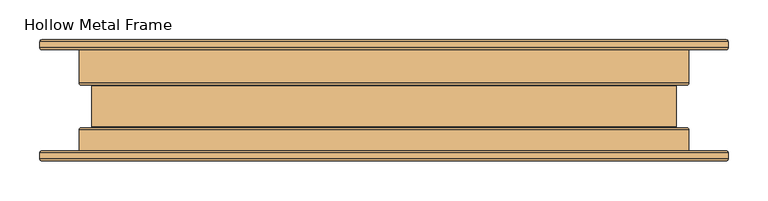
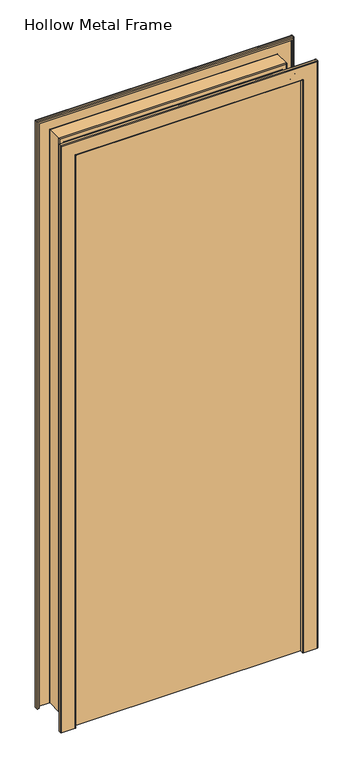
"""IFC4 building model written with IfcOpenShell, lengths in millimetres: door geometry, Hollow Metal Frame."""

import ifcopenshell
import ifcopenshell.guid

model = None  # the IFC model being written
_history = None  # IfcOwnerHistory: only IFC2X3 demands one
_inside = {}  # id of a spatial element -> (the spatial element, [elements in it])
_under = {}  # id of a project, library or spatial element -> (it, [spatial elements below it])
_declared = {}  # id of a project -> (the project, [libraries it declares])
_typed = {}  # id of a type object -> (the type object, [elements of that type])
_made_of = {}  # id of a material, layer set ... -> (it, [elements and type objects made of it])


def new_model(schema):
    """Start an empty IFC model of exactly this schema.

    Asked for "IFC4X3", IfcOpenShell would pick the latest addendum, in which some entities
    have other attributes; the version numbers below select the first issue.
    IFC2X3 requires an IfcOwnerHistory on every rooted entity: one is made here for all.
    """
    global model, _history
    if schema == "IFC4X3":
        model = ifcopenshell.file(schema_version=(4, 3, 0, 0))
    else:
        model = ifcopenshell.file(schema=schema)
    _inside.clear()
    _under.clear()
    _declared.clear()
    _typed.clear()
    _made_of.clear()
    _history = None
    if model.schema == "IFC2X3":
        org = make("IfcOrganization", Name="unknown")
        user = make(
            "IfcPersonAndOrganization",
            ThePerson=make("IfcPerson", FamilyName="unknown"),
            TheOrganization=org,
        )
        app = make(
            "IfcApplication",
            ApplicationDeveloper=org,
            Version="unknown",
            ApplicationFullName="unknown",
            ApplicationIdentifier="unknown",
        )
        _history = make(
            "IfcOwnerHistory",
            OwningUser=user,
            OwningApplication=app,
            ChangeAction="ADDED",
            CreationDate=0,
        )
    return model


def make(cls, **values):
    """One entity of the class cls with the attributes given. An attribute that is None is left unset."""
    return model.create_entity(
        cls, **{name: value for name, value in values.items() if value is not None}
    )


def rooted(cls, **values):
    """An entity with a GlobalId (a new one), such as an element, a storey or a relation."""
    return make(cls, GlobalId=ifcopenshell.guid.new(), OwnerHistory=_history, **values)


def si_unit(unit_type, name, prefix=None):
    """IfcSIUnit, for example si_unit("LENGTHUNIT", "METRE", prefix="MILLI")."""
    return make("IfcSIUnit", UnitType=unit_type, Prefix=prefix, Name=name)


def assignment(units):
    """IfcUnitAssignment: the units of a project."""
    return None if units is None else make("IfcUnitAssignment", Units=units)


def point(xyz):
    """IfcCartesianPoint."""
    return None if xyz is None else make("IfcCartesianPoint", Coordinates=xyz)


def direction(xyz):
    """IfcDirection."""
    return None if xyz is None else make("IfcDirection", DirectionRatios=xyz)


def frame(location, z_axis=None, x_axis=None):
    """IfcAxis2Placement3D, a coordinate frame: its origin and axes. An axis left out is left unset."""
    return make(
        "IfcAxis2Placement3D",
        Location=point(location),
        Axis=direction(z_axis),
        RefDirection=direction(x_axis),
    )


def origin():
    """The frame at (0, 0, 0) with its axes left unset."""
    return frame((0.0, 0.0, 0.0))


def origin_with_axes():
    """The frame at (0, 0, 0) with the z axis (0, 0, 1) and the x axis (1, 0, 0) written out."""
    return frame((0.0, 0.0, 0.0), z_axis=(0.0, 0.0, 1.0), x_axis=(1.0, 0.0, 0.0))


def place(relative_to, where):
    """IfcLocalPlacement: puts the frame where relative to a parent placement (None: the world)."""
    return make(
        "IfcLocalPlacement", PlacementRelTo=relative_to, RelativePlacement=where
    )


def context(
    kind, dimensions, precision=None, world=None, true_north=None, identifier=None
):
    """IfcGeometricRepresentationContext, for example the 3D "Model" context."""
    return make(
        "IfcGeometricRepresentationContext",
        ContextIdentifier=identifier,
        ContextType=kind,
        CoordinateSpaceDimension=dimensions,
        Precision=precision,
        WorldCoordinateSystem=world,
        TrueNorth=true_north,
    )


def project(units=None, contexts=None):
    """IfcProject with its units and contexts."""
    return rooted(
        "IfcProject",
        Name="project",
        RepresentationContexts=contexts,
        UnitsInContext=assignment(units),
    )


def spatial(cls, under=None, at=None, **own):
    """A site, building, storey or space (cls), placed at a placement, below another one or the project."""
    s = rooted(cls, ObjectPlacement=at, **own)
    if under is not None:
        _under.setdefault(under.id(), (under, []))[1].append(s)
    return s


def polyline(points):
    """IfcPolyline through the points."""
    return make("IfcPolyline", Points=[point(p) for p in points])


def circle_curve(where, radius):
    """IfcCircle in the frame where."""
    return make("IfcCircle", Position=where, Radius=radius)


def ellipse_curve(where, semi_axis1, semi_axis2):
    """IfcEllipse in the frame where."""
    return make(
        "IfcEllipse", Position=where, SemiAxis1=semi_axis1, SemiAxis2=semi_axis2
    )


def outline(outer, holes=None, kind="AREA"):
    """IfcArbitraryClosedProfileDef: a profile drawn as a closed curve; with holes, ...WithVoids."""
    if holes is None:
        return make("IfcArbitraryClosedProfileDef", ProfileType=kind, OuterCurve=outer)
    return make(
        "IfcArbitraryProfileDefWithVoids",
        ProfileType=kind,
        OuterCurve=outer,
        InnerCurves=holes,
    )


def extrude(swept, where, along, depth):
    """IfcExtrudedAreaSolid: the profile swept, set in the frame where, extruded along a direction by depth."""
    return make(
        "IfcExtrudedAreaSolid",
        SweptArea=swept,
        Position=where,
        ExtrudedDirection=direction(along),
        Depth=depth,
    )


def shape(context_of_items, identifier, shape_type, items):
    """IfcShapeRepresentation: the items that make up one representation, for example the "Body"."""
    return make(
        "IfcShapeRepresentation",
        ContextOfItems=context_of_items,
        RepresentationIdentifier=identifier,
        RepresentationType=shape_type,
        Items=items,
    )


def source(mapping_origin, context_of_items, identifier, shape_type, items):
    """IfcRepresentationMap: a shape defined once, which mapped items show again and again."""
    return make(
        "IfcRepresentationMap",
        MappingOrigin=mapping_origin,
        MappedRepresentation=shape(context_of_items, identifier, shape_type, items),
    )


def transform(
    local_origin,
    x_axis=None,
    y_axis=None,
    z_axis=None,
    scale=None,
    scale2=None,
    scale3=None,
    uniform=True,
):
    """IfcCartesianTransformationOperator3D, or its non-uniform kind. x_axis, y_axis, z_axis: its Axis1, 2, 3."""
    if uniform:
        return make(
            "IfcCartesianTransformationOperator3D",
            Axis1=direction(x_axis),
            Axis2=direction(y_axis),
            LocalOrigin=point(local_origin),
            Scale=scale,
            Axis3=direction(z_axis),
        )
    return make(
        "IfcCartesianTransformationOperator3DnonUniform",
        Axis1=direction(x_axis),
        Axis2=direction(y_axis),
        LocalOrigin=point(local_origin),
        Scale=scale,
        Axis3=direction(z_axis),
        Scale2=scale2,
        Scale3=scale3,
    )


def mapped(mapping_source, mapping_target):
    """IfcMappedItem: shows the shape of a source again, moved by a transform."""
    return make(
        "IfcMappedItem", MappingSource=mapping_source, MappingTarget=mapping_target
    )


def made_of(thing, what):
    """Note that an element or type object is made of a material, layer set ...; save() writes the relation."""
    if what is not None:
        _made_of.setdefault(what.id(), (what, []))[1].append(thing)
    return thing


def element(
    cls,
    number,
    at=None,
    inside=None,
    cuts=None,
    type_object=None,
    material=None,
    context=None,
    identifier="Body",
    shape_type=None,
    held_by="IfcProductDefinitionShape",
    body=None,
    shapes=None,
    **own,
):
    """One element of the class cls, such as IfcWall. Its Tag is "e" and its number.

    at: its placement. inside: the storey or other place that contains it. cuts: it is an
    opening in that element (IfcRelVoidsElement). A single representation is given by context,
    identifier, shape_type and body (its items); several are given by shapes. held_by: the class
    of the entity that holds the representations. save() writes the other relations.
    """
    e = rooted(cls, Tag="e%d" % number, ObjectPlacement=at, **own)
    if body is not None:
        shapes = [shape(context, identifier, shape_type, body)]
    if shapes is not None:
        e.Representation = make(held_by, Representations=shapes)
    if inside is not None:
        _inside.setdefault(inside.id(), (inside, []))[1].append(e)
    if cuts is not None:
        rooted(
            "IfcRelVoidsElement", RelatingBuildingElement=cuts, RelatedOpeningElement=e
        )
    if type_object is not None:
        _typed.setdefault(type_object.id(), (type_object, []))[1].append(e)
    return made_of(e, material)


def aggregate(whole, parts):
    """IfcRelAggregates: a whole, such as a stair, and the parts it consists of."""
    return rooted("IfcRelAggregates", RelatingObject=whole, RelatedObjects=parts)


def save(model, path):
    """Write the relations noted so far, then the file.

    IfcRelAggregates (storeys below a building ...), IfcRelContainedInSpatialStructure (elements
    in a storey), IfcRelDefinesByType, IfcRelAssociatesMaterial and IfcRelDeclares: one each for
    every whole, place, type object, material and project.
    """
    for whole, parts in _under.values():
        aggregate(whole, parts)
    for where, things in _inside.values():
        rooted(
            "IfcRelContainedInSpatialStructure",
            RelatedElements=things,
            RelatingStructure=where,
        )
    for kind, things in _typed.values():
        rooted("IfcRelDefinesByType", RelatedObjects=things, RelatingType=kind)
    for what, things in _made_of.values():
        rooted("IfcRelAssociatesMaterial", RelatedObjects=things, RelatingMaterial=what)
    for by, libraries in _declared.values():
        rooted("IfcRelDeclares", RelatingContext=by, RelatedDefinitions=libraries)
    model.write(path)


def plane_surface(at):
    """IfcPlane: the flat surface through the origin of the frame at, square to its z axis."""
    return make("IfcPlane", Position=at)


def cylinder_surface(at, radius):
    """IfcCylindricalSurface: all points at the distance radius from the z axis of the frame at."""
    return make("IfcCylindricalSurface", Position=at, Radius=radius)


def revolved_surface(curve, axis_point, axis_direction):
    """IfcSurfaceOfRevolution: the curve turned about the line through axis_point along axis_direction."""
    return make(
        "IfcSurfaceOfRevolution",
        SweptCurve=make("IfcArbitraryOpenProfileDef", ProfileType="CURVE", Curve=curve),
        AxisPosition=make("IfcAxis1Placement", Location=point(axis_point), Axis=direction(axis_direction)),
    )


def advanced_brep(points, edges, surfaces, faces):
    """IfcAdvancedBrep: a solid bounded by faces that lie on surfaces and meet in shared edges.

    An edge is (start, end): straight between two places in points (the first is 0);
    or (start, end, curve); or (start, end, curve, False) where it runs against its curve.
    A face is (place in surfaces, loops), or (place, loops, False) where it looks against
    its surface's normal. A loop lists edges by number (the first is 1), with a minus sign
    where the edge is run from its end to its start. The first loop is the outer one.
    """
    corners = [point(p) for p in points]
    vertices = [make("IfcVertexPoint", VertexGeometry=c) for c in corners]
    made = []
    for start, end, *more in edges:
        made.append(
            make(
                "IfcEdgeCurve",
                EdgeStart=vertices[start],
                EdgeEnd=vertices[end],
                EdgeGeometry=more[0] if more else make("IfcPolyline", Points=[corners[start], corners[end]]),
                SameSense=more[1] if len(more) > 1 else True,
            )
        )
    hull = []
    for where, loops, *sense in faces:
        bounds = []
        for j, loop in enumerate(loops):
            ring = [make("IfcOrientedEdge", EdgeElement=made[abs(k) - 1], Orientation=k > 0) for k in loop]
            bounds.append(
                make(
                    "IfcFaceOuterBound" if j == 0 else "IfcFaceBound",
                    Bound=make("IfcEdgeLoop", EdgeList=ring),
                    Orientation=True,
                )
            )
        hull.append(make("IfcAdvancedFace", Bounds=bounds, FaceSurface=surfaces[where], SameSense=sense[0] if sense else True))
    return make("IfcAdvancedBrep", Outer=make("IfcClosedShell", CfsFaces=hull))


def hollow_metal_frame_ce1c65a4(model_context):
    return source(origin(), model_context, "Body", "SolidModel", [
        advanced_brep(
        [(-429.22825, 63.5635, 0.0), (-431.8, 66.13525, 0.0), (-431.8, 73.66, 0.0), (-429.22825, 76.23175, 0.0), (-383.57175, 76.23175, 0.0), (-381.0, 73.66, 0.0), (-381.0, 21.68525, 0.0), (-379.984, 20.66925, 0.0), (-367.69675, 20.66925, 0.0), (-365.125, 18.0975, 0.0), (-365.125, -33.6931, 0.0), (-367.69675, -36.26485, 0.0), (-379.984, -36.26485, 0.0), (-381.0, -37.28085, 0.0), (-381.0, -73.5965, 0.0), (-383.57175, -76.16825, 0.0), (-429.22825, -76.16825, 0.0), (-431.8, -73.5965, 0.0), (-431.8, -66.07175, 0.0), (-429.22825, -63.5, 0.0), (-423.8625, -63.5, 0.0), (-423.8625, -65.05575, 0.0), (-429.22825, -65.05575, 0.0), (-430.24425, -66.07175, 0.0), (-430.24425, -73.5965, 0.0), (-429.22825, -74.6125, 0.0), (-383.57175, -74.6125, 0.0), (-382.55575, -73.5965, 0.0), (-382.55575, -37.28085, 0.0), (-379.984, -34.7091, 0.0), (-367.69675, -34.7091, 0.0), (-366.68075, -33.6931, 0.0), (-366.68075, 18.0975, 0.0), (-367.69675, 19.1135, 0.0), (-379.984, 19.1135, 0.0), (-382.55575, 21.68525, 0.0), (-382.55575, 73.66, 0.0), (-383.57175, 74.676, 0.0), (-429.22825, 74.676, 0.0), (-430.24425, 73.66, 0.0), (-430.24425, 66.13525, 0.0), (-429.22825, 65.11925, 0.0), (-423.8625, 65.11925, 0.0), (-423.8625, 63.5635, 0.0), (-429.22825, 63.5635, 2080.2282501), (-431.8, 66.13525, 2082.8000001), (-431.8, 73.66, 2082.8000001), (-429.22825, 76.23175, 2080.2282501), (429.22825, 76.23175, 2080.2282501), (429.22825, 76.23175, 0.0), (383.57175, 76.23175, 0.0), (383.57175, 76.23175, 2034.5717501), (-383.57175, 76.23175, 2034.5717501), (-381.0, 73.66, 2032.0000001), (-381.0, 21.68525, 2032.0000001), (-379.984, 20.66925, 2030.9840001), (379.984, 20.66925, 2030.9840001), (379.984, 20.66925, 0.0), (367.69675, 20.66925, 0.0), (367.69675, 20.66925, 2018.6967501), (-367.69675, 20.66925, 2018.6967501), (-365.125, 18.0975, 2016.1250001), (-365.125, -33.6931, 2016.1250001), (-367.69675, -36.26485, 2018.6967501), (367.69675, -36.26485, 2018.6967501), (367.69675, -36.26485, 0.0), (379.984, -36.26485, 0.0), (379.984, -36.26485, 2030.9840001), (-379.984, -36.26485, 2030.9840001), (-381.0, -37.28085, 2032.0000001), (-381.0, -73.5965, 2032.0000001), (-383.57175, -76.16825, 2034.5717501), (383.57175, -76.16825, 2034.5717501), (383.57175, -76.16825, 0.0), (429.22825, -76.16825, 0.0), (429.22825, -76.16825, 2080.2282501), (-429.22825, -76.16825, 2080.2282501), (-431.8, -73.5965, 2082.8000001), (-431.8, -66.07175, 2082.8000001), (-429.22825, -63.5, 2080.2282501), (429.22825, -63.5, 2080.2282501), (429.22825, -63.5, 0.0), (423.8625, -63.5, 0.0), (423.8625, -63.5, 2074.8625001), (-423.8625, -63.5, 2074.8625001), (-423.8625, -65.05575, 2074.8625001), (423.8625, -65.05575, 2074.8625001), (423.8625, -65.05575, 0.0), (429.22825, -65.05575, 0.0), (429.22825, -65.05575, 2080.2282501), (-429.22825, -65.05575, 2080.2282501), (-430.24425, -66.07175, 2081.2442501), (-430.24425, -73.5965, 2081.2442501), (-429.22825, -74.6125, 2080.2282501), (429.22825, -74.6125, 2080.2282501), (429.22825, -74.6125, 0.0), (383.57175, -74.6125, 0.0), (383.57175, -74.6125, 2034.5717501), (-383.57175, -74.6125, 2034.5717501), (-382.55575, -73.5965, 2033.5557501), (-382.55575, -37.28085, 2033.5557501), (-379.984, -34.7091, 2030.9840001), (379.984, -34.7091, 2030.9840001), (379.984, -34.7091, 0.0), (367.69675, -34.7091, 0.0), (367.69675, -34.7091, 2018.6967501), (-367.69675, -34.7091, 2018.6967501), (-366.68075, -33.6931, 2017.6807501), (-366.68075, 18.0975, 2017.6807501), (-367.69675, 19.1135, 2018.6967501), (367.69675, 19.1135, 2018.6967501), (367.69675, 19.1135, 0.0), (379.984, 19.1135, 0.0), (379.984, 19.1135, 2030.9840001), (-379.984, 19.1135, 2030.9840001), (-382.55575, 21.68525, 2033.5557501), (-382.55575, 73.66, 2033.5557501), (-383.57175, 74.676, 2034.5717501), (383.57175, 74.676, 2034.5717501), (383.57175, 74.676, 0.0), (429.22825, 74.676, 0.0), (429.22825, 74.676, 2080.2282501), (-429.22825, 74.676, 2080.2282501), (-430.24425, 73.66, 2081.2442501), (-430.24425, 66.13525, 2081.2442501), (-429.22825, 65.11925, 2080.2282501), (429.22825, 65.11925, 2080.2282501), (429.22825, 65.11925, 0.0), (423.8625, 65.11925, 0.0), (423.8625, 65.11925, 2074.8625001), (-423.8625, 65.11925, 2074.8625001), (-423.8625, 63.5635, 2074.8625001), (423.8625, 63.5635, 2074.8625001), (423.8625, 63.5635, 0.0), (429.22825, 63.5635, 0.0), (429.22825, 63.5635, 2080.2282501), (431.8, 66.13525, 2082.8000001), (431.8, 73.66, 2082.8000001), (381.0, 73.66, 2032.0000001), (381.0, 21.68525, 2032.0000001), (365.125, 18.0975, 2016.1250001), (365.125, -33.6931, 2016.1250001), (381.0, -37.28085, 2032.0000001), (381.0, -73.5965, 2032.0000001), (431.8, -73.5965, 2082.8000001), (431.8, -66.07175, 2082.8000001), (430.24425, -66.07175, 2081.2442501), (430.24425, -73.5965, 2081.2442501), (382.55575, -73.5965, 2033.5557501), (382.55575, -37.28085, 2033.5557501), (366.68075, -33.6931, 2017.6807501), (366.68075, 18.0975, 2017.6807501), (382.55575, 21.68525, 2033.5557501), (382.55575, 73.66, 2033.5557501), (430.24425, 73.66, 2081.2442501), (430.24425, 66.13525, 2081.2442501), (430.24425, 66.13525, 0.0), (430.24425, 73.66, 0.0), (382.55575, 73.66, 0.0), (382.55575, 21.68525, 0.0), (366.68075, 18.0975, 0.0), (366.68075, -33.6931, 0.0), (382.55575, -37.28085, 0.0), (382.55575, -73.5965, 0.0), (430.24425, -73.5965, 0.0), (430.24425, -66.07175, 0.0), (431.8, -66.07175, 0.0), (431.8, -73.5965, 0.0), (381.0, -73.5965, 0.0), (381.0, -37.28085, 0.0), (365.125, -33.6931, 0.0), (365.125, 18.0975, 0.0), (381.0, 21.68525, 0.0), (381.0, 73.66, 0.0), (431.8, 73.66, 0.0), (431.8, 66.13525, 0.0)],
        [
            (0, 1, circle_curve(frame((-429.22825, 66.13525, 0.0), z_axis=(0.0, 0.0, -1.0), x_axis=(0.0, -1.0, 0.0)), 2.57175)),
            (1, 2),
            (2, 3, circle_curve(frame((-429.22825, 73.66, 0.0), z_axis=(0.0, 0.0, -1.0), x_axis=(0.0, -1.0, 0.0)), 2.57175)),
            (3, 4),
            (4, 5, circle_curve(frame((-383.57175, 73.66, 0.0), z_axis=(0.0, 0.0, -1.0), x_axis=(0.0, -1.0, 0.0)), 2.57175)),
            (5, 6),
            (6, 7, circle_curve(frame((-379.984, 21.68525, 0.0), z_axis=(0.0, 0.0, 1.0), x_axis=(0.0, -1.0, 0.0)), 1.016)),
            (7, 8),
            (8, 9, circle_curve(frame((-367.69675, 18.0975, 0.0), z_axis=(0.0, 0.0, -1.0), x_axis=(0.0, -1.0, 0.0)), 2.57175)),
            (9, 10),
            (10, 11, circle_curve(frame((-367.69675, -33.6931, 0.0), z_axis=(0.0, 0.0, -1.0), x_axis=(0.0, -1.0, 0.0)), 2.57175)),
            (11, 12),
            (12, 13, circle_curve(frame((-379.984, -37.28085, 0.0), z_axis=(0.0, 0.0, 1.0), x_axis=(0.0, -1.0, 0.0)), 1.016)),
            (13, 14),
            (14, 15, circle_curve(frame((-383.57175, -73.5965, 0.0), z_axis=(0.0, 0.0, -1.0), x_axis=(0.0, -1.0, 0.0)), 2.57175)),
            (15, 16),
            (16, 17, circle_curve(frame((-429.22825, -73.5965, 0.0), z_axis=(0.0, 0.0, -1.0), x_axis=(0.0, -1.0, 0.0)), 2.57175)),
            (17, 18),
            (18, 19, circle_curve(frame((-429.22825, -66.07175, 0.0), z_axis=(0.0, 0.0, -1.0), x_axis=(0.0, -1.0, 0.0)), 2.57175)),
            (19, 20),
            (20, 21),
            (21, 22),
            (22, 23, circle_curve(frame((-429.22825, -66.07175, 0.0), z_axis=(0.0, 0.0, 1.0), x_axis=(0.0, -1.0, 0.0)), 1.016)),
            (23, 24),
            (24, 25, circle_curve(frame((-429.22825, -73.5965, 0.0), z_axis=(0.0, 0.0, 1.0), x_axis=(0.0, -1.0, 0.0)), 1.016)),
            (25, 26),
            (26, 27, circle_curve(frame((-383.57175, -73.5965, 0.0), z_axis=(0.0, 0.0, 1.0), x_axis=(0.0, -1.0, 0.0)), 1.016)),
            (27, 28),
            (28, 29, circle_curve(frame((-379.984, -37.28085, 0.0), z_axis=(0.0, 0.0, -1.0), x_axis=(0.0, -1.0, 0.0)), 2.57175)),
            (29, 30),
            (30, 31, circle_curve(frame((-367.69675, -33.6931, 0.0), z_axis=(0.0, 0.0, 1.0), x_axis=(0.0, -1.0, 0.0)), 1.016)),
            (31, 32),
            (32, 33, circle_curve(frame((-367.69675, 18.0975, 0.0), z_axis=(0.0, 0.0, 1.0), x_axis=(0.0, -1.0, 0.0)), 1.016)),
            (33, 34),
            (34, 35, circle_curve(frame((-379.984, 21.68525, 0.0), z_axis=(0.0, 0.0, -1.0), x_axis=(0.0, -1.0, 0.0)), 2.57175)),
            (35, 36),
            (36, 37, circle_curve(frame((-383.57175, 73.66, 0.0), z_axis=(0.0, 0.0, 1.0), x_axis=(0.0, -1.0, 0.0)), 1.016)),
            (37, 38),
            (38, 39, circle_curve(frame((-429.22825, 73.66, 0.0), z_axis=(0.0, 0.0, 1.0), x_axis=(0.0, -1.0, 0.0)), 1.016)),
            (39, 40),
            (40, 41, circle_curve(frame((-429.22825, 66.13525, 0.0), z_axis=(0.0, 0.0, 1.0), x_axis=(0.0, -1.0, 0.0)), 1.016)),
            (41, 42),
            (42, 43),
            (43, 0),
            (0, 44),
            (44, 45, ellipse_curve(frame((-429.22825, 66.13525, 2080.2282501), z_axis=(-0.7071067811865475, 0.0, -0.7071067811865475), x_axis=(0.7071067811865474, 0.0, -0.7071067811865476)), 3.6370037, 2.57175)),
            (45, 1),
            (45, 46),
            (46, 2),
            (46, 47, ellipse_curve(frame((-429.22825, 73.66, 2080.2282501), z_axis=(-0.7071067811865475, 0.0, -0.7071067811865475), x_axis=(0.7071067811865474, 0.0, -0.7071067811865476)), 3.6370037, 2.57175)),
            (47, 3),
            (47, 48),
            (48, 49),
            (49, 50),
            (50, 51),
            (51, 52),
            (52, 4),
            (52, 53, ellipse_curve(frame((-383.57175, 73.66, 2034.5717501), z_axis=(-0.7071067811865475, 0.0, -0.7071067811865475), x_axis=(0.7071067811865474, 0.0, -0.7071067811865476)), 3.6370037, 2.57175)),
            (53, 5),
            (53, 54),
            (54, 6),
            (54, 55, ellipse_curve(frame((-379.984, 21.68525, 2030.9840001), z_axis=(0.7071067811865475, 0.0, 0.7071067811865475), x_axis=(-0.7071067811865474, 0.0, 0.7071067811865476)), 1.436841, 1.016)),
            (55, 7),
            (55, 56),
            (56, 57),
            (57, 58),
            (58, 59),
            (59, 60),
            (60, 8),
            (60, 61, ellipse_curve(frame((-367.69675, 18.0975, 2018.6967501), z_axis=(-0.7071067811865475, 0.0, -0.7071067811865475), x_axis=(0.7071067811865474, 0.0, -0.7071067811865476)), 3.6370037, 2.57175)),
            (61, 9),
            (61, 62),
            (62, 10),
            (62, 63, ellipse_curve(frame((-367.69675, -33.6931, 2018.6967501), z_axis=(-0.7071067811865475, 0.0, -0.7071067811865475), x_axis=(0.7071067811865474, 0.0, -0.7071067811865476)), 3.6370037, 2.57175)),
            (63, 11),
            (63, 64),
            (64, 65),
            (65, 66),
            (66, 67),
            (67, 68),
            (68, 12),
            (68, 69, ellipse_curve(frame((-379.984, -37.28085, 2030.9840001), z_axis=(0.7071067811865475, 0.0, 0.7071067811865475), x_axis=(-0.7071067811865474, 0.0, 0.7071067811865476)), 1.436841, 1.016)),
            (69, 13),
            (69, 70),
            (70, 14),
            (70, 71, ellipse_curve(frame((-383.57175, -73.5965, 2034.5717501), z_axis=(-0.7071067811865475, 0.0, -0.7071067811865475), x_axis=(0.7071067811865474, 0.0, -0.7071067811865476)), 3.6370037, 2.57175)),
            (71, 15),
            (71, 72),
            (72, 73),
            (73, 74),
            (74, 75),
            (75, 76),
            (76, 16),
            (76, 77, ellipse_curve(frame((-429.22825, -73.5965, 2080.2282501), z_axis=(-0.7071067811865475, 0.0, -0.7071067811865475), x_axis=(0.7071067811865474, 0.0, -0.7071067811865476)), 3.6370037, 2.57175)),
            (77, 17),
            (77, 78),
            (78, 18),
            (78, 79, ellipse_curve(frame((-429.22825, -66.07175, 2080.2282501), z_axis=(-0.7071067811865475, 0.0, -0.7071067811865475), x_axis=(0.7071067811865474, 0.0, -0.7071067811865476)), 3.6370037, 2.57175)),
            (79, 19),
            (79, 80),
            (80, 81),
            (81, 82),
            (82, 83),
            (83, 84),
            (84, 20),
            (84, 85),
            (85, 21),
            (85, 86),
            (86, 87),
            (87, 88),
            (88, 89),
            (89, 90),
            (90, 22),
            (90, 91, ellipse_curve(frame((-429.22825, -66.07175, 2080.2282501), z_axis=(0.7071067811865475, 0.0, 0.7071067811865475), x_axis=(-0.7071067811865474, 0.0, 0.7071067811865476)), 1.436841, 1.016)),
            (91, 23),
            (91, 92),
            (92, 24),
            (92, 93, ellipse_curve(frame((-429.22825, -73.5965, 2080.2282501), z_axis=(0.7071067811865475, 0.0, 0.7071067811865475), x_axis=(-0.7071067811865474, 0.0, 0.7071067811865476)), 1.436841, 1.016)),
            (93, 25),
            (93, 94),
            (94, 95),
            (95, 96),
            (96, 97),
            (97, 98),
            (98, 26),
            (98, 99, ellipse_curve(frame((-383.57175, -73.5965, 2034.5717501), z_axis=(0.7071067811865475, 0.0, 0.7071067811865475), x_axis=(-0.7071067811865474, 0.0, 0.7071067811865476)), 1.436841, 1.016)),
            (99, 27),
            (99, 100),
            (100, 28),
            (100, 101, ellipse_curve(frame((-379.984, -37.28085, 2030.9840001), z_axis=(-0.7071067811865475, 0.0, -0.7071067811865475), x_axis=(0.7071067811865474, 0.0, -0.7071067811865476)), 3.6370037, 2.57175)),
            (101, 29),
            (101, 102),
            (102, 103),
            (103, 104),
            (104, 105),
            (105, 106),
            (106, 30),
            (106, 107, ellipse_curve(frame((-367.69675, -33.6931, 2018.6967501), z_axis=(0.7071067811865475, 0.0, 0.7071067811865475), x_axis=(-0.7071067811865474, 0.0, 0.7071067811865476)), 1.436841, 1.016)),
            (107, 31),
            (107, 108),
            (108, 32),
            (108, 109, ellipse_curve(frame((-367.69675, 18.0975, 2018.6967501), z_axis=(0.7071067811865475, 0.0, 0.7071067811865475), x_axis=(-0.7071067811865474, 0.0, 0.7071067811865476)), 1.436841, 1.016)),
            (109, 33),
            (109, 110),
            (110, 111),
            (111, 112),
            (112, 113),
            (113, 114),
            (114, 34),
            (114, 115, ellipse_curve(frame((-379.984, 21.68525, 2030.9840001), z_axis=(-0.7071067811865475, 0.0, -0.7071067811865475), x_axis=(0.7071067811865474, 0.0, -0.7071067811865476)), 3.6370037, 2.57175)),
            (115, 35),
            (115, 116),
            (116, 36),
            (116, 117, ellipse_curve(frame((-383.57175, 73.66, 2034.5717501), z_axis=(0.7071067811865475, 0.0, 0.7071067811865475), x_axis=(-0.7071067811865474, 0.0, 0.7071067811865476)), 1.436841, 1.016)),
            (117, 37),
            (117, 118),
            (118, 119),
            (119, 120),
            (120, 121),
            (121, 122),
            (122, 38),
            (122, 123, ellipse_curve(frame((-429.22825, 73.66, 2080.2282501), z_axis=(0.7071067811865475, 0.0, 0.7071067811865475), x_axis=(-0.7071067811865474, 0.0, 0.7071067811865476)), 1.436841, 1.016)),
            (123, 39),
            (123, 124),
            (124, 40),
            (124, 125, ellipse_curve(frame((-429.22825, 66.13525, 2080.2282501), z_axis=(0.7071067811865475, 0.0, 0.7071067811865475), x_axis=(-0.7071067811865474, 0.0, 0.7071067811865476)), 1.436841, 1.016)),
            (125, 41),
            (125, 126),
            (126, 127),
            (127, 128),
            (128, 129),
            (129, 130),
            (130, 42),
            (130, 131),
            (131, 43),
            (131, 132),
            (132, 133),
            (133, 134),
            (134, 135),
            (135, 44),
            (135, 136, ellipse_curve(frame((429.22825, 66.13525, 2080.2282501), z_axis=(-0.7071067811865475, 0.0, 0.7071067811865475), x_axis=(-0.7071067811865476, 0.0, -0.7071067811865474)), 3.6370037, 2.57175)),
            (136, 45),
            (136, 137),
            (137, 46),
            (137, 48, ellipse_curve(frame((429.22825, 73.66, 2080.2282501), z_axis=(-0.7071067811865475, 0.0, 0.7071067811865475), x_axis=(-0.7071067811865476, 0.0, -0.7071067811865474)), 3.6370037, 2.57175)),
            (51, 138, ellipse_curve(frame((383.57175, 73.66, 2034.5717501), z_axis=(-0.7071067811865475, 0.0, 0.7071067811865475), x_axis=(-0.7071067811865476, 0.0, -0.7071067811865474)), 3.6370037, 2.57175)),
            (138, 53),
            (138, 139),
            (139, 54),
            (139, 56, ellipse_curve(frame((379.984, 21.68525, 2030.9840001), z_axis=(0.7071067811865475, 0.0, -0.7071067811865475), x_axis=(0.7071067811865476, 0.0, 0.7071067811865474)), 1.436841, 1.016)),
            (59, 140, ellipse_curve(frame((367.69675, 18.0975, 2018.6967501), z_axis=(-0.7071067811865475, 0.0, 0.7071067811865475), x_axis=(-0.7071067811865476, 0.0, -0.7071067811865474)), 3.6370037, 2.57175)),
            (140, 61),
            (140, 141),
            (141, 62),
            (141, 64, ellipse_curve(frame((367.69675, -33.6931, 2018.6967501), z_axis=(-0.7071067811865475, 0.0, 0.7071067811865475), x_axis=(-0.7071067811865476, 0.0, -0.7071067811865474)), 3.6370037, 2.57175)),
            (67, 142, ellipse_curve(frame((379.984, -37.28085, 2030.9840001), z_axis=(0.7071067811865475, 0.0, -0.7071067811865475), x_axis=(0.7071067811865476, 0.0, 0.7071067811865474)), 1.436841, 1.016)),
            (142, 69),
            (142, 143),
            (143, 70),
            (143, 72, ellipse_curve(frame((383.57175, -73.5965, 2034.5717501), z_axis=(-0.7071067811865475, 0.0, 0.7071067811865475), x_axis=(-0.7071067811865476, 0.0, -0.7071067811865474)), 3.6370037, 2.57175)),
            (75, 144, ellipse_curve(frame((429.22825, -73.5965, 2080.2282501), z_axis=(-0.7071067811865475, 0.0, 0.7071067811865475), x_axis=(-0.7071067811865476, 0.0, -0.7071067811865474)), 3.6370037, 2.57175)),
            (144, 77),
            (144, 145),
            (145, 78),
            (145, 80, ellipse_curve(frame((429.22825, -66.07175, 2080.2282501), z_axis=(-0.7071067811865475, 0.0, 0.7071067811865475), x_axis=(-0.7071067811865476, 0.0, -0.7071067811865474)), 3.6370037, 2.57175)),
            (83, 86),
            (89, 146, ellipse_curve(frame((429.22825, -66.07175, 2080.2282501), z_axis=(0.7071067811865475, 0.0, -0.7071067811865475), x_axis=(0.7071067811865476, 0.0, 0.7071067811865474)), 1.436841, 1.016)),
            (146, 91),
            (146, 147),
            (147, 92),
            (147, 94, ellipse_curve(frame((429.22825, -73.5965, 2080.2282501), z_axis=(0.7071067811865475, 0.0, -0.7071067811865475), x_axis=(0.7071067811865476, 0.0, 0.7071067811865474)), 1.436841, 1.016)),
            (97, 148, ellipse_curve(frame((383.57175, -73.5965, 2034.5717501), z_axis=(0.7071067811865475, 0.0, -0.7071067811865475), x_axis=(0.7071067811865476, 0.0, 0.7071067811865474)), 1.436841, 1.016)),
            (148, 99),
            (148, 149),
            (149, 100),
            (149, 102, ellipse_curve(frame((379.984, -37.28085, 2030.9840001), z_axis=(-0.7071067811865475, 0.0, 0.7071067811865475), x_axis=(-0.7071067811865476, 0.0, -0.7071067811865474)), 3.6370037, 2.57175)),
            (105, 150, ellipse_curve(frame((367.69675, -33.6931, 2018.6967501), z_axis=(0.7071067811865475, 0.0, -0.7071067811865475), x_axis=(0.7071067811865476, 0.0, 0.7071067811865474)), 1.436841, 1.016)),
            (150, 107),
            (150, 151),
            (151, 108),
            (151, 110, ellipse_curve(frame((367.69675, 18.0975, 2018.6967501), z_axis=(0.7071067811865475, 0.0, -0.7071067811865475), x_axis=(0.7071067811865476, 0.0, 0.7071067811865474)), 1.436841, 1.016)),
            (113, 152, ellipse_curve(frame((379.984, 21.68525, 2030.9840001), z_axis=(-0.7071067811865475, 0.0, 0.7071067811865475), x_axis=(-0.7071067811865476, 0.0, -0.7071067811865474)), 3.6370037, 2.57175)),
            (152, 115),
            (152, 153),
            (153, 116),
            (153, 118, ellipse_curve(frame((383.57175, 73.66, 2034.5717501), z_axis=(0.7071067811865475, 0.0, -0.7071067811865475), x_axis=(0.7071067811865476, 0.0, 0.7071067811865474)), 1.436841, 1.016)),
            (121, 154, ellipse_curve(frame((429.22825, 73.66, 2080.2282501), z_axis=(0.7071067811865475, 0.0, -0.7071067811865475), x_axis=(0.7071067811865476, 0.0, 0.7071067811865474)), 1.436841, 1.016)),
            (154, 123),
            (154, 155),
            (155, 124),
            (155, 126, ellipse_curve(frame((429.22825, 66.13525, 2080.2282501), z_axis=(0.7071067811865475, 0.0, -0.7071067811865475), x_axis=(0.7071067811865476, 0.0, 0.7071067811865474)), 1.436841, 1.016)),
            (129, 132),
            (133, 128),
            (127, 156, circle_curve(frame((429.22825, 66.13525, 0.0), z_axis=(0.0, 0.0, 1.0), x_axis=(0.0, -1.0, 0.0)), 1.016)),
            (156, 157),
            (157, 120, circle_curve(frame((429.22825, 73.66, 0.0), z_axis=(0.0, 0.0, 1.0), x_axis=(0.0, -1.0, 0.0)), 1.016)),
            (119, 158, circle_curve(frame((383.57175, 73.66, 0.0), z_axis=(0.0, 0.0, 1.0), x_axis=(0.0, -1.0, 0.0)), 1.016)),
            (158, 159),
            (159, 112, circle_curve(frame((379.984, 21.68525, 0.0), z_axis=(0.0, 0.0, -1.0), x_axis=(0.0, -1.0, 0.0)), 2.57175)),
            (111, 160, circle_curve(frame((367.69675, 18.0975, 0.0), z_axis=(0.0, 0.0, 1.0), x_axis=(0.0, -1.0, 0.0)), 1.016)),
            (160, 161),
            (161, 104, circle_curve(frame((367.69675, -33.6931, 0.0), z_axis=(0.0, 0.0, 1.0), x_axis=(0.0, -1.0, 0.0)), 1.016)),
            (103, 162, circle_curve(frame((379.984, -37.28085, 0.0), z_axis=(0.0, 0.0, -1.0), x_axis=(0.0, -1.0, 0.0)), 2.57175)),
            (162, 163),
            (163, 96, circle_curve(frame((383.57175, -73.5965, 0.0), z_axis=(0.0, 0.0, 1.0), x_axis=(0.0, -1.0, 0.0)), 1.016)),
            (95, 164, circle_curve(frame((429.22825, -73.5965, 0.0), z_axis=(0.0, 0.0, 1.0), x_axis=(0.0, -1.0, 0.0)), 1.016)),
            (164, 165),
            (165, 88, circle_curve(frame((429.22825, -66.07175, 0.0), z_axis=(0.0, 0.0, 1.0), x_axis=(0.0, -1.0, 0.0)), 1.016)),
            (87, 82),
            (81, 166, circle_curve(frame((429.22825, -66.07175, 0.0), z_axis=(0.0, 0.0, -1.0), x_axis=(0.0, -1.0, 0.0)), 2.57175)),
            (166, 167),
            (167, 74, circle_curve(frame((429.22825, -73.5965, 0.0), z_axis=(0.0, 0.0, -1.0), x_axis=(0.0, -1.0, 0.0)), 2.57175)),
            (73, 168, circle_curve(frame((383.57175, -73.5965, 0.0), z_axis=(0.0, 0.0, -1.0), x_axis=(0.0, -1.0, 0.0)), 2.57175)),
            (168, 169),
            (169, 66, circle_curve(frame((379.984, -37.28085, 0.0), z_axis=(0.0, 0.0, 1.0), x_axis=(0.0, -1.0, 0.0)), 1.016)),
            (65, 170, circle_curve(frame((367.69675, -33.6931, 0.0), z_axis=(0.0, 0.0, -1.0), x_axis=(0.0, -1.0, 0.0)), 2.57175)),
            (170, 171),
            (171, 58, circle_curve(frame((367.69675, 18.0975, 0.0), z_axis=(0.0, 0.0, -1.0), x_axis=(0.0, -1.0, 0.0)), 2.57175)),
            (57, 172, circle_curve(frame((379.984, 21.68525, 0.0), z_axis=(0.0, 0.0, 1.0), x_axis=(0.0, -1.0, 0.0)), 1.016)),
            (172, 173),
            (173, 50, circle_curve(frame((383.57175, 73.66, 0.0), z_axis=(0.0, 0.0, -1.0), x_axis=(0.0, -1.0, 0.0)), 2.57175)),
            (49, 174, circle_curve(frame((429.22825, 73.66, 0.0), z_axis=(0.0, 0.0, -1.0), x_axis=(0.0, -1.0, 0.0)), 2.57175)),
            (174, 175),
            (175, 134, circle_curve(frame((429.22825, 66.13525, 0.0), z_axis=(0.0, 0.0, -1.0), x_axis=(0.0, -1.0, 0.0)), 2.57175)),
            (175, 136),
            (174, 137),
            (173, 138),
            (172, 139),
            (171, 140),
            (170, 141),
            (169, 142),
            (168, 143),
            (167, 144),
            (166, 145),
            (165, 146),
            (164, 147),
            (163, 148),
            (162, 149),
            (161, 150),
            (160, 151),
            (159, 152),
            (158, 153),
            (157, 154),
            (156, 155),
        ],
        [
            plane_surface(frame((-392.1125, -63.5, 0.0), z_axis=(0.0, 0.0, -1.0), x_axis=(1.0, 0.0, 0.0))),
            cylinder_surface(frame((-429.22825, 66.13525, 0.0), z_axis=(0.0, 0.0, -1.0), x_axis=(0.0, -1.0, 0.0)), 2.57175),
            plane_surface(frame((-431.8, 66.13525, 0.0), z_axis=(-1.0, 0.0, 0.0), x_axis=(0.0, 0.0, 1.0))),
            cylinder_surface(frame((-429.22825, 73.66, 0.0), z_axis=(0.0, 0.0, -1.0), x_axis=(0.0, -1.0, 0.0)), 2.57175),
            plane_surface(frame((-429.22825, 76.23175, 0.0), z_axis=(0.0, 1.0, 0.0), x_axis=(0.0, 0.0, 1.0))),
            cylinder_surface(frame((-383.57175, 73.66, 0.0), z_axis=(0.0, 0.0, -1.0), x_axis=(0.0, -1.0, 0.0)), 2.57175),
            plane_surface(frame((-381.0, 73.66, 0.0), z_axis=(1.0, 0.0, 0.0), x_axis=(0.0, 0.0, 1.0))),
            revolved_surface(polyline([(-379.984, 20.669249999999998, 2032.0000001145868), (-379.984, 20.669249999999998, 0.0)]), (-379.984, 21.68525, 0.0), (0.0, 0.0, 1.0)),
            plane_surface(frame((-379.984, 20.66925, 0.0), z_axis=(0.0, 1.0, 0.0), x_axis=(0.0, 0.0, 1.0))),
            cylinder_surface(frame((-367.69675, 18.0975, 0.0), z_axis=(0.0, 0.0, -1.0), x_axis=(0.0, -1.0, 0.0)), 2.57175),
            plane_surface(frame((-365.125, 18.0975, 0.0), z_axis=(1.0, 0.0, 0.0), x_axis=(0.0, 0.0, 1.0))),
            cylinder_surface(frame((-367.69675, -33.6931, 0.0), z_axis=(0.0, 0.0, -1.0), x_axis=(0.0, -1.0, 0.0)), 2.57175),
            plane_surface(frame((-367.69675, -36.26485, 0.0), z_axis=(0.0, -1.0, 0.0), x_axis=(0.0, 0.0, 1.0))),
            revolved_surface(polyline([(-379.984, -38.29685, 2032.0000001145868), (-379.984, -38.29685, 0.0)]), (-379.984, -37.28085, 0.0), (0.0, 0.0, 1.0)),
            plane_surface(frame((-381.0, -37.28085, 0.0), z_axis=(1.0, 0.0, 0.0), x_axis=(0.0, 0.0, 1.0))),
            cylinder_surface(frame((-383.57175, -73.5965, 0.0), z_axis=(0.0, 0.0, -1.0), x_axis=(0.0, -1.0, 0.0)), 2.57175),
            plane_surface(frame((-383.57175, -76.16825, 0.0), z_axis=(0.0, -1.0, 0.0), x_axis=(0.0, 0.0, 1.0))),
            cylinder_surface(frame((-429.22825, -73.5965, 0.0), z_axis=(0.0, 0.0, -1.0), x_axis=(0.0, -1.0, 0.0)), 2.57175),
            plane_surface(frame((-431.8, -73.5965, 0.0), z_axis=(-1.0, 0.0, 0.0), x_axis=(0.0, 0.0, 1.0))),
            cylinder_surface(frame((-429.22825, -66.07175, 0.0), z_axis=(0.0, 0.0, -1.0), x_axis=(0.0, -1.0, 0.0)), 2.57175),
            plane_surface(frame((-429.22825, -63.5, 0.0), z_axis=(0.0, 1.0, 0.0), x_axis=(0.0, 0.0, 1.0))),
            plane_surface(frame((-423.8625, -63.5, 0.0), z_axis=(1.0, 0.0, 0.0), x_axis=(0.0, 0.0, 1.0))),
            plane_surface(frame((-423.8625, -65.05575, 0.0), z_axis=(0.0, -1.0, 0.0), x_axis=(0.0, 0.0, 1.0))),
            revolved_surface(polyline([(-429.22825, -67.08775, 2081.244250114587), (-429.22825, -67.08775, 0.0)]), (-429.22825, -66.07175, 0.0), (0.0, 0.0, 1.0)),
            plane_surface(frame((-430.24425, -66.07175, 0.0), z_axis=(1.0, 0.0, 0.0), x_axis=(0.0, 0.0, 1.0))),
            revolved_surface(polyline([(-429.22825, -74.61250000000001, 2081.244250114587), (-429.22825, -74.61250000000001, 0.0)]), (-429.22825, -73.5965, 0.0), (0.0, 0.0, 1.0)),
            plane_surface(frame((-429.22825, -74.6125, 0.0), z_axis=(0.0, 1.0, 0.0), x_axis=(0.0, 0.0, 1.0))),
            revolved_surface(polyline([(-383.57175, -74.61250000000001, 2035.5877501145867), (-383.57175, -74.61250000000001, 0.0)]), (-383.57175, -73.5965, 0.0), (0.0, 0.0, 1.0)),
            plane_surface(frame((-382.55575, -73.5965, 0.0), z_axis=(-1.0, 0.0, 0.0), x_axis=(0.0, 0.0, 1.0))),
            cylinder_surface(frame((-379.984, -37.28085, 0.0), z_axis=(0.0, 0.0, -1.0), x_axis=(0.0, -1.0, 0.0)), 2.57175),
            plane_surface(frame((-379.984, -34.7091, 0.0), z_axis=(0.0, 1.0, 0.0), x_axis=(0.0, 0.0, 1.0))),
            revolved_surface(polyline([(-367.69675, -34.7091, 2019.7127501145867), (-367.69675, -34.7091, 0.0)]), (-367.69675, -33.6931, 0.0), (0.0, 0.0, 1.0)),
            plane_surface(frame((-366.68075, -33.6931, 0.0), z_axis=(-1.0, 0.0, 0.0), x_axis=(0.0, 0.0, 1.0))),
            revolved_surface(polyline([(-367.69675, 17.0815, 2019.7127501145867), (-367.69675, 17.0815, 0.0)]), (-367.69675, 18.0975, 0.0), (0.0, 0.0, 1.0)),
            plane_surface(frame((-367.69675, 19.1135, 0.0), z_axis=(0.0, -1.0, 0.0), x_axis=(0.0, 0.0, 1.0))),
            cylinder_surface(frame((-379.984, 21.68525, 0.0), z_axis=(0.0, 0.0, -1.0), x_axis=(0.0, -1.0, 0.0)), 2.57175),
            plane_surface(frame((-382.55575, 21.68525, 0.0), z_axis=(-1.0, 0.0, 0.0), x_axis=(0.0, 0.0, 1.0))),
            revolved_surface(polyline([(-383.57175, 72.64399999999999, 2035.5877501145867), (-383.57175, 72.64399999999999, 0.0)]), (-383.57175, 73.66, 0.0), (0.0, 0.0, 1.0)),
            plane_surface(frame((-383.57175, 74.676, 0.0), z_axis=(0.0, -1.0, 0.0), x_axis=(0.0, 0.0, 1.0))),
            revolved_surface(polyline([(-429.22825, 72.64399999999999, 2081.244250114587), (-429.22825, 72.64399999999999, 0.0)]), (-429.22825, 73.66, 0.0), (0.0, 0.0, 1.0)),
            plane_surface(frame((-430.24425, 73.66, 0.0), z_axis=(1.0, 0.0, 0.0), x_axis=(0.0, 0.0, 1.0))),
            revolved_surface(polyline([(-429.22825, 65.11925, 2081.244250114587), (-429.22825, 65.11925, 0.0)]), (-429.22825, 66.13525, 0.0), (0.0, 0.0, 1.0)),
            plane_surface(frame((-429.22825, 65.11925, 0.0), z_axis=(0.0, 1.0, 0.0), x_axis=(0.0, 0.0, 1.0))),
            plane_surface(frame((-423.8625, 65.11925, 0.0), z_axis=(1.0, 0.0, 0.0), x_axis=(0.0, 0.0, 1.0))),
            plane_surface(frame((-423.8625, 63.5635, 0.0), z_axis=(0.0, -1.0, 0.0), x_axis=(0.0, 0.0, 1.0))),
            cylinder_surface(frame((-392.1125, 66.13525, 2080.2282501), z_axis=(-1.0, 0.0, 0.0), x_axis=(0.0, -1.0, 0.0)), 2.57175),
            plane_surface(frame((-431.8, 66.13525, 2082.8000001), z_axis=(0.0, 0.0, 1.0), x_axis=(1.0, 0.0, 0.0))),
            cylinder_surface(frame((-392.1125, 73.66, 2080.2282501), z_axis=(-1.0, 0.0, 0.0), x_axis=(0.0, -1.0, 0.0)), 2.57175),
            cylinder_surface(frame((-392.1125, 73.66, 2034.5717501), z_axis=(-1.0, 0.0, 0.0), x_axis=(0.0, -1.0, 0.0)), 2.57175),
            plane_surface(frame((-381.0, 73.66, 2032.0000001), z_axis=(0.0, 0.0, -1.0), x_axis=(1.0, 0.0, 0.0))),
            revolved_surface(polyline([(381.0000000145869, 20.669249999999998, 2030.9840001), (-381.0000000145868, 20.669249999999998, 2030.9840001)]), (-392.1125, 21.68525, 2030.9840001), (1.0, 0.0, 0.0)),
            cylinder_surface(frame((-392.1125, 18.0975, 2018.6967501), z_axis=(-1.0, 0.0, 0.0), x_axis=(0.0, -1.0, 0.0)), 2.57175),
            plane_surface(frame((-365.125, 18.0975, 2016.1250001), z_axis=(0.0, 0.0, -1.0), x_axis=(1.0, 0.0, 0.0))),
            cylinder_surface(frame((-392.1125, -33.6931, 2018.6967501), z_axis=(-1.0, 0.0, 0.0), x_axis=(0.0, -1.0, 0.0)), 2.57175),
            revolved_surface(polyline([(381.0000000145869, -38.29685, 2030.9840001), (-381.0000000145868, -38.29685, 2030.9840001)]), (-392.1125, -37.28085, 2030.9840001), (1.0, 0.0, 0.0)),
            plane_surface(frame((-381.0, -37.28085, 2032.0000001), z_axis=(0.0, 0.0, -1.0), x_axis=(1.0, 0.0, 0.0))),
            cylinder_surface(frame((-392.1125, -73.5965, 2034.5717501), z_axis=(-1.0, 0.0, 0.0), x_axis=(0.0, -1.0, 0.0)), 2.57175),
            cylinder_surface(frame((-392.1125, -73.5965, 2080.2282501), z_axis=(-1.0, 0.0, 0.0), x_axis=(0.0, -1.0, 0.0)), 2.57175),
            plane_surface(frame((-431.8, -73.5965, 2082.8000001), z_axis=(0.0, 0.0, 1.0), x_axis=(1.0, 0.0, 0.0))),
            cylinder_surface(frame((-392.1125, -66.07175, 2080.2282501), z_axis=(-1.0, 0.0, 0.0), x_axis=(0.0, -1.0, 0.0)), 2.57175),
            plane_surface(frame((-423.8625, -63.5, 2074.8625001), z_axis=(0.0, 0.0, -1.0), x_axis=(1.0, 0.0, 0.0))),
            revolved_surface(polyline([(430.24425001458695, -67.08775, 2080.2282501), (-430.24425001458684, -67.08775, 2080.2282501)]), (-392.1125, -66.07175, 2080.2282501), (1.0, 0.0, 0.0)),
            plane_surface(frame((-430.24425, -66.07175, 2081.2442501), z_axis=(0.0, 0.0, -1.0), x_axis=(1.0, 0.0, 0.0))),
            revolved_surface(polyline([(430.24425001458695, -74.61250000000001, 2080.2282501), (-430.24425001458684, -74.61250000000001, 2080.2282501)]), (-392.1125, -73.5965, 2080.2282501), (1.0, 0.0, 0.0)),
            revolved_surface(polyline([(384.5877500145869, -74.61250000000001, 2034.5717501), (-384.58775001458685, -74.61250000000001, 2034.5717501)]), (-392.1125, -73.5965, 2034.5717501), (1.0, 0.0, 0.0)),
            plane_surface(frame((-382.55575, -73.5965, 2033.5557501), z_axis=(0.0, 0.0, 1.0), x_axis=(1.0, 0.0, 0.0))),
            cylinder_surface(frame((-392.1125, -37.28085, 2030.9840001), z_axis=(-1.0, 0.0, 0.0), x_axis=(0.0, -1.0, 0.0)), 2.57175),
            revolved_surface(polyline([(368.7127500145869, -34.7091, 2018.6967501), (-368.71275001458685, -34.7091, 2018.6967501)]), (-392.1125, -33.6931, 2018.6967501), (1.0, 0.0, 0.0)),
            plane_surface(frame((-366.68075, -33.6931, 2017.6807501), z_axis=(0.0, 0.0, 1.0), x_axis=(1.0, 0.0, 0.0))),
            revolved_surface(polyline([(368.7127500145869, 17.0815, 2018.6967501), (-368.71275001458685, 17.0815, 2018.6967501)]), (-392.1125, 18.0975, 2018.6967501), (1.0, 0.0, 0.0)),
            cylinder_surface(frame((-392.1125, 21.68525, 2030.9840001), z_axis=(-1.0, 0.0, 0.0), x_axis=(0.0, -1.0, 0.0)), 2.57175),
            plane_surface(frame((-382.55575, 21.68525, 2033.5557501), z_axis=(0.0, 0.0, 1.0), x_axis=(1.0, 0.0, 0.0))),
            revolved_surface(polyline([(384.5877500145869, 72.64399999999999, 2034.5717501), (-384.58775001458685, 72.64399999999999, 2034.5717501)]), (-392.1125, 73.66, 2034.5717501), (1.0, 0.0, 0.0)),
            revolved_surface(polyline([(430.24425001458695, 72.64399999999999, 2080.2282501), (-430.24425001458684, 72.64399999999999, 2080.2282501)]), (-392.1125, 73.66, 2080.2282501), (1.0, 0.0, 0.0)),
            plane_surface(frame((-430.24425, 73.66, 2081.2442501), z_axis=(0.0, 0.0, -1.0), x_axis=(1.0, 0.0, 0.0))),
            revolved_surface(polyline([(430.24425001458695, 65.11925, 2080.2282501), (-430.24425001458684, 65.11925, 2080.2282501)]), (-392.1125, 66.13525, 2080.2282501), (1.0, 0.0, 0.0)),
            plane_surface(frame((-423.8625, 65.11925, 2074.8625001), z_axis=(0.0, 0.0, -1.0), x_axis=(1.0, 0.0, 0.0))),
            plane_surface(frame((392.1125, -63.5, 0.0), z_axis=(0.0, 0.0, -1.0), x_axis=(-1.0, 0.0, 0.0))),
            cylinder_surface(frame((429.22825, 66.13525, 2043.1125001), z_axis=(0.0, 0.0, 1.0), x_axis=(0.0, -1.0, 0.0)), 2.57175),
            plane_surface(frame((431.8, 66.13525, 2082.8000001), z_axis=(1.0, 0.0, 0.0), x_axis=(0.0, 0.0, -1.0))),
            cylinder_surface(frame((429.22825, 73.66, 2043.1125001), z_axis=(0.0, 0.0, 1.0), x_axis=(0.0, -1.0, 0.0)), 2.57175),
            cylinder_surface(frame((383.57175, 73.66, 2043.1125001), z_axis=(0.0, 0.0, 1.0), x_axis=(0.0, -1.0, 0.0)), 2.57175),
            plane_surface(frame((381.0, 73.66, 2032.0000001), z_axis=(-1.0, 0.0, 0.0), x_axis=(0.0, 0.0, -1.0))),
            revolved_surface(polyline([(379.984, 20.669249999999998, 0.0), (379.984, 20.669249999999998, 2032.0000001145868)]), (379.984, 21.68525, 2043.1125001), (0.0, 0.0, -1.0)),
            cylinder_surface(frame((367.69675, 18.0975, 2043.1125001), z_axis=(0.0, 0.0, 1.0), x_axis=(0.0, -1.0, 0.0)), 2.57175),
            plane_surface(frame((365.125, 18.0975, 2016.1250001), z_axis=(-1.0, 0.0, 0.0), x_axis=(0.0, 0.0, -1.0))),
            cylinder_surface(frame((367.69675, -33.6931, 2043.1125001), z_axis=(0.0, 0.0, 1.0), x_axis=(0.0, -1.0, 0.0)), 2.57175),
            revolved_surface(polyline([(379.984, -38.29685, 0.0), (379.984, -38.29685, 2032.0000001145868)]), (379.984, -37.28085, 2043.1125001), (0.0, 0.0, -1.0)),
            plane_surface(frame((381.0, -37.28085, 2032.0000001), z_axis=(-1.0, 0.0, 0.0), x_axis=(0.0, 0.0, -1.0))),
            cylinder_surface(frame((383.57175, -73.5965, 2043.1125001), z_axis=(0.0, 0.0, 1.0), x_axis=(0.0, -1.0, 0.0)), 2.57175),
            cylinder_surface(frame((429.22825, -73.5965, 2043.1125001), z_axis=(0.0, 0.0, 1.0), x_axis=(0.0, -1.0, 0.0)), 2.57175),
            plane_surface(frame((431.8, -73.5965, 2082.8000001), z_axis=(1.0, 0.0, 0.0), x_axis=(0.0, 0.0, -1.0))),
            cylinder_surface(frame((429.22825, -66.07175, 2043.1125001), z_axis=(0.0, 0.0, 1.0), x_axis=(0.0, -1.0, 0.0)), 2.57175),
            plane_surface(frame((423.8625, -63.5, 2074.8625001), z_axis=(-1.0, 0.0, 0.0), x_axis=(0.0, 0.0, -1.0))),
            revolved_surface(polyline([(429.22825, -67.08775, 0.0), (429.22825, -67.08775, 2081.244250114587)]), (429.22825, -66.07175, 2043.1125001), (0.0, 0.0, -1.0)),
            plane_surface(frame((430.24425, -66.07175, 2081.2442501), z_axis=(-1.0, 0.0, 0.0), x_axis=(0.0, 0.0, -1.0))),
            revolved_surface(polyline([(429.22825, -74.61250000000001, 0.0), (429.22825, -74.61250000000001, 2081.244250114587)]), (429.22825, -73.5965, 2043.1125001), (0.0, 0.0, -1.0)),
            revolved_surface(polyline([(383.57175, -74.61250000000001, 0.0), (383.57175, -74.61250000000001, 2035.5877501145867)]), (383.57175, -73.5965, 2043.1125001), (0.0, 0.0, -1.0)),
            plane_surface(frame((382.55575, -73.5965, 2033.5557501), z_axis=(1.0, 0.0, 0.0), x_axis=(0.0, 0.0, -1.0))),
            cylinder_surface(frame((379.984, -37.28085, 2043.1125001), z_axis=(0.0, 0.0, 1.0), x_axis=(0.0, -1.0, 0.0)), 2.57175),
            revolved_surface(polyline([(367.69675, -34.7091, 0.0), (367.69675, -34.7091, 2019.7127501145867)]), (367.69675, -33.6931, 2043.1125001), (0.0, 0.0, -1.0)),
            plane_surface(frame((366.68075, -33.6931, 2017.6807501), z_axis=(1.0, 0.0, 0.0), x_axis=(0.0, 0.0, -1.0))),
            revolved_surface(polyline([(367.69675, 17.0815, 0.0), (367.69675, 17.0815, 2019.7127501145867)]), (367.69675, 18.0975, 2043.1125001), (0.0, 0.0, -1.0)),
            cylinder_surface(frame((379.984, 21.68525, 2043.1125001), z_axis=(0.0, 0.0, 1.0), x_axis=(0.0, -1.0, 0.0)), 2.57175),
            plane_surface(frame((382.55575, 21.68525, 2033.5557501), z_axis=(1.0, 0.0, 0.0), x_axis=(0.0, 0.0, -1.0))),
            revolved_surface(polyline([(383.57175, 72.64399999999999, 0.0), (383.57175, 72.64399999999999, 2035.5877501145867)]), (383.57175, 73.66, 2043.1125001), (0.0, 0.0, -1.0)),
            revolved_surface(polyline([(429.22825, 72.64399999999999, 0.0), (429.22825, 72.64399999999999, 2081.244250114587)]), (429.22825, 73.66, 2043.1125001), (0.0, 0.0, -1.0)),
            plane_surface(frame((430.24425, 73.66, 2081.2442501), z_axis=(-1.0, 0.0, 0.0), x_axis=(0.0, 0.0, -1.0))),
            revolved_surface(polyline([(429.22825, 65.11925, 0.0), (429.22825, 65.11925, 2081.244250114587)]), (429.22825, 66.13525, 2043.1125001), (0.0, 0.0, -1.0)),
            plane_surface(frame((423.8625, 65.11925, 2074.8625001), z_axis=(-1.0, 0.0, 0.0), x_axis=(0.0, 0.0, -1.0))),
        ],
        [
            (0, [[1, 2, 3, 4, 5, 6, 7, 8, 9, 10, 11, 12, 13, 14, 15, 16, 17, 18, 19, 20, 21, 22, 23, 24, 25, 26, 27, 28, 29, 30, 31, 32, 33, 34, 35, 36, 37, 38, 39, 40, 41, 42, 43, 44]]),
            (1, [[-1, 45, 46, 47]]),
            (2, [[-2, -47, 48, 49]]),
            (3, [[-3, -49, 50, 51]]),
            (4, [[-4, -51, 52, 53, 54, 55, 56, 57]]),
            (5, [[-5, -57, 58, 59]]),
            (6, [[-6, -59, 60, 61]]),
            (7, [[-7, -61, 62, 63]]),
            (8, [[-8, -63, 64, 65, 66, 67, 68, 69]]),
            (9, [[-9, -69, 70, 71]]),
            (10, [[-10, -71, 72, 73]]),
            (11, [[-11, -73, 74, 75]]),
            (12, [[-12, -75, 76, 77, 78, 79, 80, 81]]),
            (13, [[-13, -81, 82, 83]]),
            (14, [[-14, -83, 84, 85]]),
            (15, [[-15, -85, 86, 87]]),
            (16, [[-16, -87, 88, 89, 90, 91, 92, 93]]),
            (17, [[-17, -93, 94, 95]]),
            (18, [[-18, -95, 96, 97]]),
            (19, [[-19, -97, 98, 99]]),
            (20, [[-20, -99, 100, 101, 102, 103, 104, 105]]),
            (21, [[-21, -105, 106, 107]]),
            (22, [[-22, -107, 108, 109, 110, 111, 112, 113]]),
            (23, [[-23, -113, 114, 115]]),
            (24, [[-24, -115, 116, 117]]),
            (25, [[-25, -117, 118, 119]]),
            (26, [[-26, -119, 120, 121, 122, 123, 124, 125]]),
            (27, [[-27, -125, 126, 127]]),
            (28, [[-28, -127, 128, 129]]),
            (29, [[-29, -129, 130, 131]]),
            (30, [[-30, -131, 132, 133, 134, 135, 136, 137]]),
            (31, [[-31, -137, 138, 139]]),
            (32, [[-32, -139, 140, 141]]),
            (33, [[-33, -141, 142, 143]]),
            (34, [[-34, -143, 144, 145, 146, 147, 148, 149]]),
            (35, [[-35, -149, 150, 151]]),
            (36, [[-36, -151, 152, 153]]),
            (37, [[-37, -153, 154, 155]]),
            (38, [[-38, -155, 156, 157, 158, 159, 160, 161]]),
            (39, [[-39, -161, 162, 163]]),
            (40, [[-40, -163, 164, 165]]),
            (41, [[-41, -165, 166, 167]]),
            (42, [[-42, -167, 168, 169, 170, 171, 172, 173]]),
            (43, [[-43, -173, 174, 175]]),
            (44, [[-44, -175, 176, 177, 178, 179, 180, -45]]),
            (45, [[-46, -180, 181, 182]]),
            (46, [[-48, -182, 183, 184]]),
            (47, [[-50, -184, 185, -52]]),
            (48, [[-58, -56, 186, 187]]),
            (49, [[-60, -187, 188, 189]]),
            (50, [[-62, -189, 190, -64]]),
            (51, [[-70, -68, 191, 192]]),
            (52, [[-72, -192, 193, 194]]),
            (53, [[-74, -194, 195, -76]]),
            (54, [[-82, -80, 196, 197]]),
            (55, [[-84, -197, 198, 199]]),
            (56, [[-86, -199, 200, -88]]),
            (57, [[-94, -92, 201, 202]]),
            (58, [[-96, -202, 203, 204]]),
            (59, [[-98, -204, 205, -100]]),
            (60, [[-106, -104, 206, -108]]),
            (61, [[-114, -112, 207, 208]]),
            (62, [[-116, -208, 209, 210]]),
            (63, [[-118, -210, 211, -120]]),
            (64, [[-126, -124, 212, 213]]),
            (65, [[-128, -213, 214, 215]]),
            (66, [[-130, -215, 216, -132]]),
            (67, [[-138, -136, 217, 218]]),
            (68, [[-140, -218, 219, 220]]),
            (69, [[-142, -220, 221, -144]]),
            (70, [[-150, -148, 222, 223]]),
            (71, [[-152, -223, 224, 225]]),
            (72, [[-154, -225, 226, -156]]),
            (73, [[-162, -160, 227, 228]]),
            (74, [[-164, -228, 229, 230]]),
            (75, [[-166, -230, 231, -168]]),
            (76, [[-174, -172, 232, -176]]),
            (77, [[-178, 233, -170, 234, 235, 236, -158, 237, 238, 239, -146, 240, 241, 242, -134, 243, 244, 245, -122, 246, 247, 248, -110, 249, -102, 250, 251, 252, -90, 253, 254, 255, -78, 256, 257, 258, -66, 259, 260, 261, -54, 262, 263, 264]]),
            (78, [[-181, -179, -264, 265]]),
            (79, [[-183, -265, -263, 266]]),
            (80, [[-185, -266, -262, -53]]),
            (81, [[-186, -55, -261, 267]]),
            (82, [[-188, -267, -260, 268]]),
            (83, [[-190, -268, -259, -65]]),
            (84, [[-191, -67, -258, 269]]),
            (85, [[-193, -269, -257, 270]]),
            (86, [[-195, -270, -256, -77]]),
            (87, [[-196, -79, -255, 271]]),
            (88, [[-198, -271, -254, 272]]),
            (89, [[-200, -272, -253, -89]]),
            (90, [[-201, -91, -252, 273]]),
            (91, [[-203, -273, -251, 274]]),
            (92, [[-205, -274, -250, -101]]),
            (93, [[-206, -103, -249, -109]]),
            (94, [[-207, -111, -248, 275]]),
            (95, [[-209, -275, -247, 276]]),
            (96, [[-211, -276, -246, -121]]),
            (97, [[-212, -123, -245, 277]]),
            (98, [[-214, -277, -244, 278]]),
            (99, [[-216, -278, -243, -133]]),
            (100, [[-217, -135, -242, 279]]),
            (101, [[-219, -279, -241, 280]]),
            (102, [[-221, -280, -240, -145]]),
            (103, [[-222, -147, -239, 281]]),
            (104, [[-224, -281, -238, 282]]),
            (105, [[-226, -282, -237, -157]]),
            (106, [[-227, -159, -236, 283]]),
            (107, [[-229, -283, -235, 284]]),
            (108, [[-231, -284, -234, -169]]),
            (109, [[-232, -171, -233, -177]]),
        ],
    ),
        extrude(outline(polyline([(379.44425, -37.28085), (379.44425, -63.5), (-379.44425, -63.5), (-379.44425, -37.28085), (379.44425, -37.28085)])), origin_with_axes(), (0.0, 0.0, 1.0), 2032.0000001),
    ])


if __name__ == "__main__":
    model = new_model("IFC4")
    model_context = context("Model", 3, world=origin())
    ifc_project = project(units=[si_unit("LENGTHUNIT", "METRE", prefix="MILLI")], contexts=[model_context])
    site = spatial("IfcSite", under=ifc_project)
    building = spatial("IfcBuilding", under=site)
    placement = place(None, origin())
    hollow_metal_frame_shape = hollow_metal_frame_ce1c65a4(model_context)
    element("IfcDoor", 1, ObjectType="Hollow Metal Frame : 2'-6\"W x 6'-8\"H", at=placement, inside=building, context=model_context, shape_type="MappedRepresentation", body=[
        mapped(hollow_metal_frame_shape, transform((0.0, 0.0, 0.0), x_axis=(1.0, 0.0, 0.0), y_axis=(0.0, 1.0, 0.0), z_axis=(0.0, 0.0, 1.0))),
    ])
    save(model, "model.ifc")

# Revit data of these elements
# Type "Hollow Metal Frame : 2'-6\"W x 6'-8\"H"
#   Type Mark = "p"
#   Product Page URL = ""
#   Product Name = ""
#   Product Documentation Link = ""
#   Material = ""
#   DS_Hardware_Set_(SFT) = ""
#   DS_Frame_Type_(SFT) = ""
#   DS_Fire_Rating_(SFT) = ""
#   DS_Door_Type_(SFT) = ""
#   Analytic Construction = "<None>"
#   Frame Projection Ext. = 0' - 1"
#   Frame Projection Int. = 0' - 1"
#   Frame Width = 0' - 3"
#   Height = 6' - 8"
#   Width = 2' - 6"
#   Non-Kerfed = yes
#   Kerfed = no
#   Hollow Metal Casing = Metal-Dunbarton_Doors-White
#   Flush Door = Metal-Dunbarton_Doors-Aluminum
#   DS_Frame_Material_(SFT) = none
#   DS_Door_Material_(SFT) = none
#   URL = ""
#   Model = ""
#   Manufacturer = ""
#   Function = (empty or 0)
#   Wall Closure = (empty or 0)
#   Description = (empty or 0)
# Element 1 (IfcDoor, "Hollow Metal Frame : 2'-6\"W x 6'-8\"H")
#   Materials on its faces: "Metal-Dunbarton_Doors-White", "Metal-Dunbarton_Doors-Aluminum"
# Materials
#   "Metal-Dunbarton_Doors-White": class "Miscellaneous", colour RGB 230 233 236, transparency 0
#   "Metal-Dunbarton_Doors-Aluminum": class "System", colour RGB 143 142 141, transparency 0
